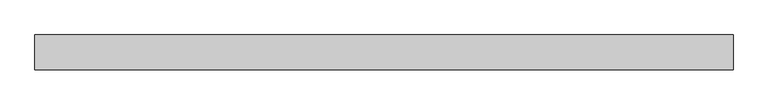
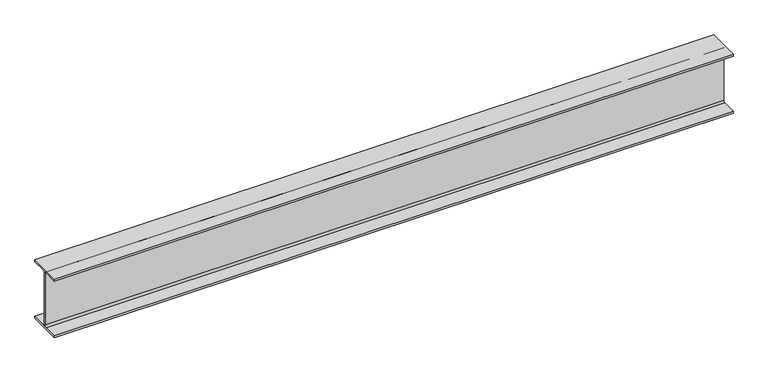
"""IFC4 building model written with IfcOpenShell, lengths in millimetres: beam geometry, Old_Steel Beam_H-KSD3502 : H_SB_ASB_H-200×200x8x12."""

from ifc_helpers import new_model, si_unit, point, frame, frame_2d, origin, place, context, project, spatial, polyline, circle_curve, trimmed, segment, composite_curve, outline, extrude, source, transform, mapped, element, save


def beam_87a33373(model_context):
    return source(origin(), model_context, "Body", "SweptSolid", [
        extrude(outline(composite_curve([segment(polyline([(82.5, -141.5), (82.5, -151.7), (-82.5, -151.7), (-82.5, -141.5), (-11.9, -141.5)]), True, "CONTINUOUS"), segment(trimmed(circle_curve(frame_2d((-11.9, -132.6)), 8.9), [point((-11.9, -141.5))], [point((-3.0, -132.6))], True, "CARTESIAN"), True, "CONTINUOUS"), segment(polyline([(-3.0, -132.6), (-3.0, 132.6)]), True, "CONTINUOUS"), segment(trimmed(circle_curve(frame_2d((-11.9, 132.6)), 8.9), [point((-3.0, 132.6))], [point((-11.9, 141.5))], True, "CARTESIAN"), True, "CONTINUOUS"), segment(polyline([(-11.9, 141.5), (-82.5, 141.5), (-82.5, 151.7), (82.5, 151.7), (82.5, 141.5), (11.9, 141.5)]), True, "CONTINUOUS"), segment(trimmed(circle_curve(frame_2d((11.9, 132.6)), 8.9), [point((11.9, 141.5))], [point((3.0, 132.6))], True, "CARTESIAN"), True, "CONTINUOUS"), segment(polyline([(3.0, 132.6), (3.0, -132.6)]), True, "CONTINUOUS"), segment(trimmed(circle_curve(frame_2d((11.9, -132.6)), 8.9), [point((3.0, -132.6))], [point((11.9, -141.5))], True, "CARTESIAN"), True, "CONTINUOUS"), segment(polyline([(11.9, -141.5), (82.5, -141.5)]), True, "CONTINUOUS")], self_intersect=False)), frame((-1611.7677924, 0.0, 0.0), z_axis=(1.0, 0.0, 0.0), x_axis=(0.0, 1.0, 0.0)), (0.0, 0.0, 1.0), 3310.7044425),
    ])


if __name__ == "__main__":
    model = new_model("IFC4")
    model_context = context("Model", 3, world=origin())
    ifc_project = project(units=[si_unit("LENGTHUNIT", "METRE", prefix="MILLI")], contexts=[model_context])
    site = spatial("IfcSite", under=ifc_project)
    building = spatial("IfcBuilding", under=site)
    placement = place(None, origin())
    beam_shape = beam_87a33373(model_context)
    element("IfcBeam", 1, ObjectType="Old_Steel Beam_H-KSD3502 : H_SB_ASB_H-200×200x8x12", at=placement, inside=building, context=model_context, shape_type="MappedRepresentation", body=[
        mapped(beam_shape, transform((0.0, 0.0, 0.0), x_axis=(1.0, 0.0, 0.0), y_axis=(0.0, 1.0, 0.0), z_axis=(0.0, 0.0, 1.0))),
    ])
    save(model, "model.ifc")

# Revit data of these elements
# Type "Old_Steel Beam_H-KSD3502 : H_SB_ASB_H-200×200x8x12"
#   Width = 20.0 cm
#   Web Thickness = 0.8 cm
#   Web Fillet = 1.3 cm
#   Warping Constant = 141376.0 cm⁶
#   Torsional Moment of Inertia = 26.2485 cm⁴
#   Torsional Modulus = 1.0 cm³
#   Section Area = 63.53 cm²
#   Plastic Modulus weak axis = 244.0 cm³
#   Plastic Modulus strong axis = 525.0 cm³
#   Perimeter = 1.16 m²/m
#   Nominal Weight = 49.90 kgf/m
#   Moment of Inertia weak axis = 1600.00 cm⁴
#   Moment of Inertia strong axis = 4720.00 cm⁴
#   Height = 20.0 cm
#   Flange Thickness = 1.2 cm
#   Elastic Modulus weak axis = 160.0 cm³
#   Elastic Modulus strong axis = 472.0 cm³
#   Centroid Vertical = 10.0 cm
#   Centroid Horizontal = 10.0 cm
#   Length [instance default] = 1.5240 m
#   Structural Material [instance default] = Steel, 45-345
#   Assembly Code = ""
# Element 1 (IfcBeam, "Old_Steel Beam_H-KSD3502 : H_SB_ASB_H-200×200x8x12")
#   Structural Material = none
# Materials
#   "Steel, 45-345": class "Metal", colour RGB 189 187 185, transparency 0, Description = "Steel 345 MPa", Cost = 0
